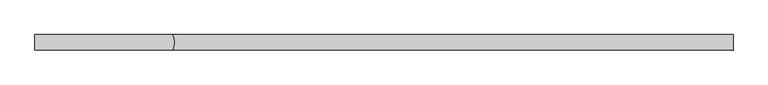
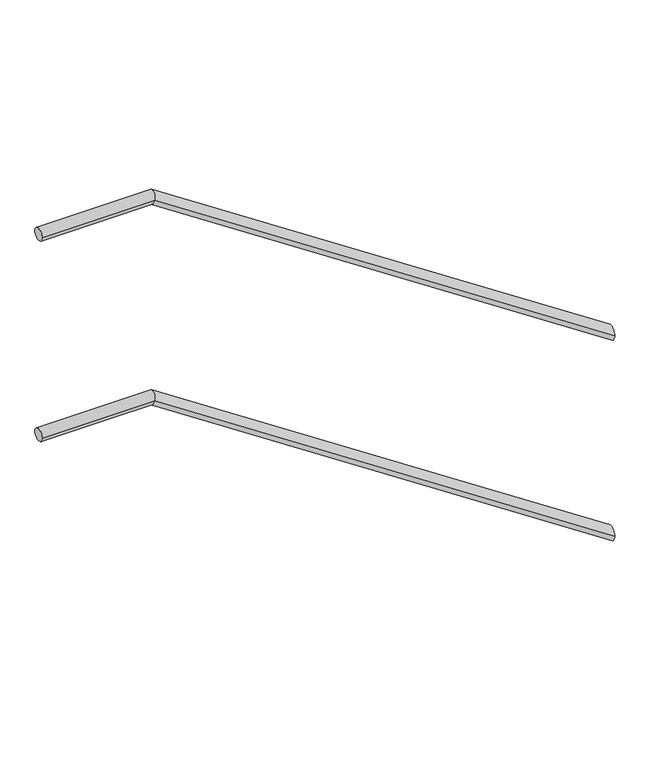
"""IFC4 building model written with IfcOpenShell, lengths in millimetres: railing geometry."""

from ifc_helpers import new_model, si_unit, frame, origin, place, context, project, spatial, circle_curve, ellipse_curve, source, transform, mapped, element, save
from ifc_brep_helpers import plane_surface, cylinder_surface, advanced_brep


def railing_d88b3958(model_context):
    return source(origin(), model_context, "Body", "AdvancedBrep", [
        advanced_brep(
        [(48078.2332408, 6875.4306666, 910.5875748), (48078.2332408, 6845.4306666, 910.5875748), (46993.7216539, 6875.4306666, 1627.8571429), (46993.7216539, 6845.4306666, 1627.8571429), (46728.2332408, 6875.4306666, 1627.8571429), (46728.2332408, 6845.4306666, 1627.8571429)],
        [
            (0, 1, ellipse_curve(frame((48078.2332408, 6860.4306666, 910.5875748), z_axis=(1.0, 0.0, 0.0), x_axis=(0.0, 0.0, -1.0)), 17.9838538, 15.0)),
            (1, 0, ellipse_curve(frame((48078.2332408, 6860.4306666, 910.5875748), z_axis=(1.0, 0.0, 0.0), x_axis=(0.0, 0.0, -1.0)), 17.9838538, 15.0)),
            (0, 2),
            (2, 3, ellipse_curve(frame((46993.7216539, 6860.4306666, 1627.8571429), z_axis=(0.9576224501515418, 0.0, -0.28802646226650325), x_axis=(-0.288026462266502, 0.0, -0.9576224501515423)), 15.6637932, 15.0)),
            (3, 1),
            (3, 2, ellipse_curve(frame((46993.7216539, 6860.4306666, 1627.8571429), z_axis=(0.9576224501515418, 0.0, -0.28802646226650325), x_axis=(-0.288026462266502, 0.0, -0.9576224501515423)), 15.6637932, 15.0)),
            (4, 5, circle_curve(frame((46728.2332408, 6860.4306666, 1627.8571429), z_axis=(-1.0, 0.0, 0.0), x_axis=(0.0, -1.0, 0.0)), 15.0)),
            (5, 4, circle_curve(frame((46728.2332408, 6860.4306666, 1627.8571429), z_axis=(-1.0, 0.0, 0.0), x_axis=(0.0, -1.0, 0.0)), 15.0)),
            (2, 4),
            (5, 3),
        ],
        [
            plane_surface(frame((48078.2332408, 6860.4306666, 928.5714286), z_axis=(1.0, 0.0, 0.0), x_axis=(0.0, -1.0, 0.0))),
            cylinder_surface(frame((48069.9586226, 6860.4306666, 916.0602059), z_axis=(0.8340815140684851, 0.0, -0.5516412130082591), x_axis=(0.0, -1.0, 0.0)), 15.0),
            plane_surface(frame((46728.2332408, 6860.4306666, 1642.8571429), z_axis=(-1.0, 0.0, 0.0), x_axis=(0.0, -1.0, 0.0))),
            cylinder_surface(frame((46998.2332408, 6860.4306666, 1627.8571429), z_axis=(1.0, 0.0, 0.0), x_axis=(0.0, -1.0, 0.0)), 15.0),
        ],
        [
            (0, [[1, 2]]),
            (1, [[-1, 3, 4, 5]]),
            (1, [[-2, -5, 6, -3]]),
            (2, [[7, 8]]),
            (3, [[-4, 9, -8, 10]]),
            (3, [[-6, -10, -7, -9]]),
        ],
    ),
        advanced_brep(
        [(48078.2332408, 6875.4306666, 1410.5875748), (48078.2332408, 6845.4306666, 1410.5875748), (46993.7216539, 6875.4306666, 2127.8571429), (46993.7216539, 6845.4306666, 2127.8571429), (46728.2332408, 6875.4306666, 2127.8571429), (46728.2332408, 6845.4306666, 2127.8571429)],
        [
            (0, 1, ellipse_curve(frame((48078.2332408, 6860.4306666, 1410.5875748), z_axis=(1.0, 0.0, 0.0), x_axis=(0.0, 0.0, -1.0)), 17.9838538, 15.0)),
            (1, 0, ellipse_curve(frame((48078.2332408, 6860.4306666, 1410.5875748), z_axis=(1.0, 0.0, 0.0), x_axis=(0.0, 0.0, -1.0)), 17.9838538, 15.0)),
            (0, 2),
            (2, 3, ellipse_curve(frame((46993.7216539, 6860.4306666, 2127.8571429), z_axis=(0.9576224501515418, 0.0, -0.28802646226650325), x_axis=(-0.288026462266502, 0.0, -0.9576224501515423)), 15.6637932, 15.0)),
            (3, 1),
            (3, 2, ellipse_curve(frame((46993.7216539, 6860.4306666, 2127.8571429), z_axis=(0.9576224501515418, 0.0, -0.28802646226650325), x_axis=(-0.288026462266502, 0.0, -0.9576224501515423)), 15.6637932, 15.0)),
            (4, 5, circle_curve(frame((46728.2332408, 6860.4306666, 2127.8571429), z_axis=(-1.0, 0.0, 0.0), x_axis=(0.0, -1.0, 0.0)), 15.0)),
            (5, 4, circle_curve(frame((46728.2332408, 6860.4306666, 2127.8571429), z_axis=(-1.0, 0.0, 0.0), x_axis=(0.0, -1.0, 0.0)), 15.0)),
            (2, 4),
            (5, 3),
        ],
        [
            plane_surface(frame((48078.2332408, 6860.4306666, 1428.5714286), z_axis=(1.0, 0.0, 0.0), x_axis=(0.0, -1.0, 0.0))),
            cylinder_surface(frame((48069.9586226, 6860.4306666, 1416.0602059), z_axis=(0.8340815140684851, 0.0, -0.5516412130082591), x_axis=(0.0, -1.0, 0.0)), 15.0),
            plane_surface(frame((46728.2332408, 6860.4306666, 2142.8571429), z_axis=(-1.0, 0.0, 0.0), x_axis=(0.0, -1.0, 0.0))),
            cylinder_surface(frame((46998.2332408, 6860.4306666, 2127.8571429), z_axis=(1.0, 0.0, 0.0), x_axis=(0.0, -1.0, 0.0)), 15.0),
        ],
        [
            (0, [[1, 2]]),
            (1, [[-1, 3, 4, 5]]),
            (1, [[-2, -5, 6, -3]]),
            (2, [[7, 8]]),
            (3, [[-4, 9, -8, 10]]),
            (3, [[-6, -10, -7, -9]]),
        ],
    ),
    ])


if __name__ == "__main__":
    model = new_model("IFC4")
    model_context = context("Model", 3, world=origin())
    ifc_project = project(units=[si_unit("LENGTHUNIT", "METRE", prefix="MILLI")], contexts=[model_context])
    site = spatial("IfcSite", under=ifc_project)
    building = spatial("IfcBuilding", under=site)
    placement = place(None, origin())
    railing_shape = railing_d88b3958(model_context)
    element("IfcRailing", 1, at=placement, inside=building, context=model_context, shape_type="MappedRepresentation", body=[
        mapped(railing_shape, transform((0.0, 0.0, 0.0), x_axis=(1.0, 0.0, 0.0), y_axis=(0.0, 1.0, 0.0), z_axis=(0.0, 0.0, 1.0))),
    ])
    save(model, "model.ifc")
